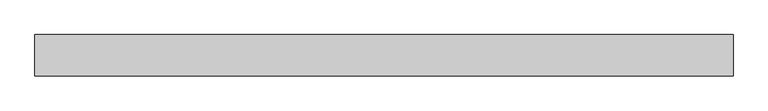
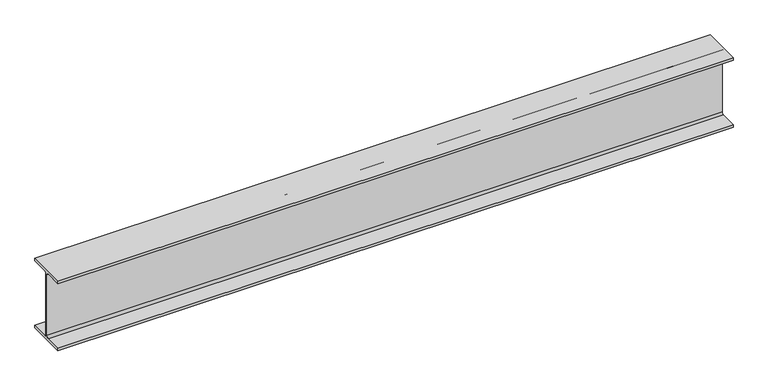
"""IFC4 building model written with IfcOpenShell, lengths in millimetres: beam geometry, Old_Steel Beam_H-KSD3502 : H_SB_ASB_H-250×125x6x9."""

from ifc_helpers import new_model, si_unit, point, frame, frame_2d, origin, place, context, project, spatial, polyline, circle_curve, trimmed, segment, composite_curve, outline, extrude, source, transform, mapped, element, save


def beam_a34f7ceb(model_context):
    return source(origin(), model_context, "Body", "SweptSolid", [
        extrude(outline(composite_curve([segment(polyline([(82.5, -141.5), (82.5, -151.7), (-82.5, -151.7), (-82.5, -141.5), (-11.9, -141.5)]), True, "CONTINUOUS"), segment(trimmed(circle_curve(frame_2d((-11.9, -132.6)), 8.9), [point((-11.9, -141.5))], [point((-3.0, -132.6))], True, "CARTESIAN"), True, "CONTINUOUS"), segment(polyline([(-3.0, -132.6), (-3.0, 132.6)]), True, "CONTINUOUS"), segment(trimmed(circle_curve(frame_2d((-11.9, 132.6)), 8.9), [point((-3.0, 132.6))], [point((-11.9, 141.5))], True, "CARTESIAN"), True, "CONTINUOUS"), segment(polyline([(-11.9, 141.5), (-82.5, 141.5), (-82.5, 151.7), (82.5, 151.7), (82.5, 141.5), (11.9, 141.5)]), True, "CONTINUOUS"), segment(trimmed(circle_curve(frame_2d((11.9, 132.6)), 8.9), [point((11.9, 141.5))], [point((3.0, 132.6))], True, "CARTESIAN"), True, "CONTINUOUS"), segment(polyline([(3.0, 132.6), (3.0, -132.6)]), True, "CONTINUOUS"), segment(trimmed(circle_curve(frame_2d((11.9, -132.6)), 8.9), [point((3.0, -132.6))], [point((11.9, -141.5))], True, "CARTESIAN"), True, "CONTINUOUS"), segment(polyline([(11.9, -141.5), (82.5, -141.5)]), True, "CONTINUOUS")], self_intersect=False)), frame((-1382.3488581, 0.0, 0.0), z_axis=(1.0, 0.0, 0.0), x_axis=(0.0, 1.0, 0.0)), (0.0, 0.0, 1.0), 2794.6488581),
    ])


if __name__ == "__main__":
    model = new_model("IFC4")
    model_context = context("Model", 3, world=origin())
    ifc_project = project(units=[si_unit("LENGTHUNIT", "METRE", prefix="MILLI")], contexts=[model_context])
    site = spatial("IfcSite", under=ifc_project)
    building = spatial("IfcBuilding", under=site)
    placement = place(None, origin())
    beam_shape = beam_a34f7ceb(model_context)
    element("IfcBeam", 1, ObjectType="Old_Steel Beam_H-KSD3502 : H_SB_ASB_H-250×125x6x9", at=placement, inside=building, context=model_context, shape_type="MappedRepresentation", body=[
        mapped(beam_shape, transform((0.0, 0.0, 0.0), x_axis=(1.0, 0.0, 0.0), y_axis=(0.0, 1.0, 0.0), z_axis=(0.0, 0.0, 1.0))),
    ])
    save(model, "model.ifc")

# Revit data of these elements
# Type "Old_Steel Beam_H-KSD3502 : H_SB_ASB_H-250×125x6x9"
#   Width = 12.5 cm
#   Web Thickness = 0.6 cm
#   Web Fillet = 1.2 cm
#   Warping Constant = 42539.8 cm⁶
#   Torsional Moment of Inertia = 7.8102 cm⁴
#   Torsional Modulus = 1.0 cm³
#   Section Area = 37.66 cm²
#   Plastic Modulus weak axis = 73.1 cm³
#   Plastic Modulus strong axis = 366.0 cm³
#   Perimeter = 0.97 m²/m
#   Nominal Weight = 29.60 kgf/m
#   Moment of Inertia weak axis = 294.00 cm⁴
#   Moment of Inertia strong axis = 4050.00 cm⁴
#   Height = 25.0 cm
#   Flange Thickness = 0.9 cm
#   Elastic Modulus weak axis = 47.0 cm³
#   Elastic Modulus strong axis = 324.0 cm³
#   Centroid Vertical = 12.5 cm
#   Centroid Horizontal = 6.25 cm
#   Length [instance default] = 1.5240 m
#   Structural Material [instance default] = Steel, 45-345
#   Assembly Code = ""
# Element 1 (IfcBeam, "Old_Steel Beam_H-KSD3502 : H_SB_ASB_H-250×125x6x9")
#   Structural Material = none
# Materials
#   "Steel, 45-345": class "Metal", colour RGB 189 187 185, transparency 0, Description = "Steel 345 MPa", Cost = 0
